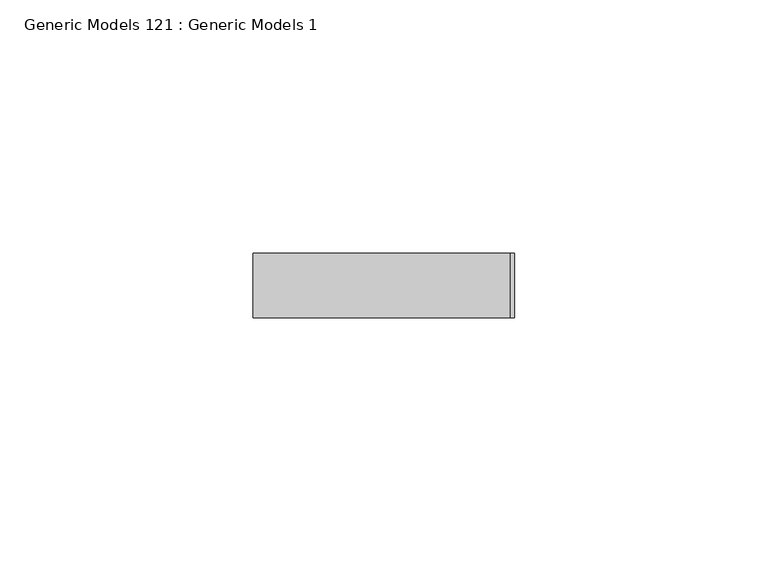
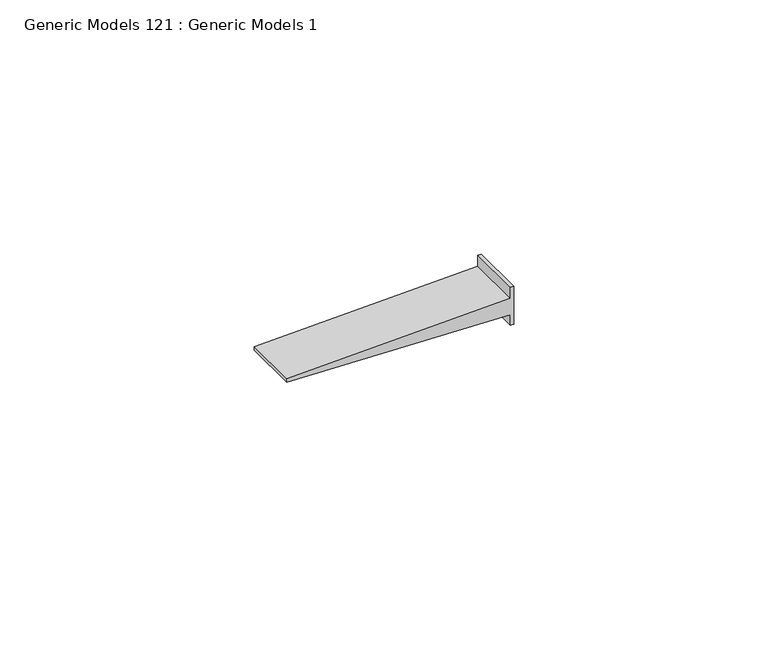
"""IFC4 building model written with IfcOpenShell, lengths in millimetres: proxy geometry, Generic Models 121 : Generic Models 1."""

import ifcopenshell
import ifcopenshell.guid

model = None  # the IFC model being written
_history = None  # IfcOwnerHistory: only IFC2X3 demands one
_inside = {}  # id of a spatial element -> (the spatial element, [elements in it])
_under = {}  # id of a project, library or spatial element -> (it, [spatial elements below it])
_declared = {}  # id of a project -> (the project, [libraries it declares])
_typed = {}  # id of a type object -> (the type object, [elements of that type])
_made_of = {}  # id of a material, layer set ... -> (it, [elements and type objects made of it])


def new_model(schema):
    """Start an empty IFC model of exactly this schema.

    Asked for "IFC4X3", IfcOpenShell would pick the latest addendum, in which some entities
    have other attributes; the version numbers below select the first issue.
    IFC2X3 requires an IfcOwnerHistory on every rooted entity: one is made here for all.
    """
    global model, _history
    if schema == "IFC4X3":
        model = ifcopenshell.file(schema_version=(4, 3, 0, 0))
    else:
        model = ifcopenshell.file(schema=schema)
    _inside.clear()
    _under.clear()
    _declared.clear()
    _typed.clear()
    _made_of.clear()
    _history = None
    if model.schema == "IFC2X3":
        org = make("IfcOrganization", Name="unknown")
        user = make(
            "IfcPersonAndOrganization",
            ThePerson=make("IfcPerson", FamilyName="unknown"),
            TheOrganization=org,
        )
        app = make(
            "IfcApplication",
            ApplicationDeveloper=org,
            Version="unknown",
            ApplicationFullName="unknown",
            ApplicationIdentifier="unknown",
        )
        _history = make(
            "IfcOwnerHistory",
            OwningUser=user,
            OwningApplication=app,
            ChangeAction="ADDED",
            CreationDate=0,
        )
    return model


def make(cls, **values):
    """One entity of the class cls with the attributes given. An attribute that is None is left unset."""
    return model.create_entity(
        cls, **{name: value for name, value in values.items() if value is not None}
    )


def rooted(cls, **values):
    """An entity with a GlobalId (a new one), such as an element, a storey or a relation."""
    return make(cls, GlobalId=ifcopenshell.guid.new(), OwnerHistory=_history, **values)


def si_unit(unit_type, name, prefix=None):
    """IfcSIUnit, for example si_unit("LENGTHUNIT", "METRE", prefix="MILLI")."""
    return make("IfcSIUnit", UnitType=unit_type, Prefix=prefix, Name=name)


def assignment(units):
    """IfcUnitAssignment: the units of a project."""
    return None if units is None else make("IfcUnitAssignment", Units=units)


def point(xyz):
    """IfcCartesianPoint."""
    return None if xyz is None else make("IfcCartesianPoint", Coordinates=xyz)


def direction(xyz):
    """IfcDirection."""
    return None if xyz is None else make("IfcDirection", DirectionRatios=xyz)


def frame(location, z_axis=None, x_axis=None):
    """IfcAxis2Placement3D, a coordinate frame: its origin and axes. An axis left out is left unset."""
    return make(
        "IfcAxis2Placement3D",
        Location=point(location),
        Axis=direction(z_axis),
        RefDirection=direction(x_axis),
    )


def origin():
    """The frame at (0, 0, 0) with its axes left unset."""
    return frame((0.0, 0.0, 0.0))


def place(relative_to, where):
    """IfcLocalPlacement: puts the frame where relative to a parent placement (None: the world)."""
    return make(
        "IfcLocalPlacement", PlacementRelTo=relative_to, RelativePlacement=where
    )


def context(
    kind, dimensions, precision=None, world=None, true_north=None, identifier=None
):
    """IfcGeometricRepresentationContext, for example the 3D "Model" context."""
    return make(
        "IfcGeometricRepresentationContext",
        ContextIdentifier=identifier,
        ContextType=kind,
        CoordinateSpaceDimension=dimensions,
        Precision=precision,
        WorldCoordinateSystem=world,
        TrueNorth=true_north,
    )


def project(units=None, contexts=None):
    """IfcProject with its units and contexts."""
    return rooted(
        "IfcProject",
        Name="project",
        RepresentationContexts=contexts,
        UnitsInContext=assignment(units),
    )


def spatial(cls, under=None, at=None, **own):
    """A site, building, storey or space (cls), placed at a placement, below another one or the project."""
    s = rooted(cls, ObjectPlacement=at, **own)
    if under is not None:
        _under.setdefault(under.id(), (under, []))[1].append(s)
    return s


def polyline(points):
    """IfcPolyline through the points."""
    return make("IfcPolyline", Points=[point(p) for p in points])


def outline(outer, holes=None, kind="AREA"):
    """IfcArbitraryClosedProfileDef: a profile drawn as a closed curve; with holes, ...WithVoids."""
    if holes is None:
        return make("IfcArbitraryClosedProfileDef", ProfileType=kind, OuterCurve=outer)
    return make(
        "IfcArbitraryProfileDefWithVoids",
        ProfileType=kind,
        OuterCurve=outer,
        InnerCurves=holes,
    )


def extrude(swept, where, along, depth):
    """IfcExtrudedAreaSolid: the profile swept, set in the frame where, extruded along a direction by depth."""
    return make(
        "IfcExtrudedAreaSolid",
        SweptArea=swept,
        Position=where,
        ExtrudedDirection=direction(along),
        Depth=depth,
    )


def shape(context_of_items, identifier, shape_type, items):
    """IfcShapeRepresentation: the items that make up one representation, for example the "Body"."""
    return make(
        "IfcShapeRepresentation",
        ContextOfItems=context_of_items,
        RepresentationIdentifier=identifier,
        RepresentationType=shape_type,
        Items=items,
    )


def source(mapping_origin, context_of_items, identifier, shape_type, items):
    """IfcRepresentationMap: a shape defined once, which mapped items show again and again."""
    return make(
        "IfcRepresentationMap",
        MappingOrigin=mapping_origin,
        MappedRepresentation=shape(context_of_items, identifier, shape_type, items),
    )


def transform(
    local_origin,
    x_axis=None,
    y_axis=None,
    z_axis=None,
    scale=None,
    scale2=None,
    scale3=None,
    uniform=True,
):
    """IfcCartesianTransformationOperator3D, or its non-uniform kind. x_axis, y_axis, z_axis: its Axis1, 2, 3."""
    if uniform:
        return make(
            "IfcCartesianTransformationOperator3D",
            Axis1=direction(x_axis),
            Axis2=direction(y_axis),
            LocalOrigin=point(local_origin),
            Scale=scale,
            Axis3=direction(z_axis),
        )
    return make(
        "IfcCartesianTransformationOperator3DnonUniform",
        Axis1=direction(x_axis),
        Axis2=direction(y_axis),
        LocalOrigin=point(local_origin),
        Scale=scale,
        Axis3=direction(z_axis),
        Scale2=scale2,
        Scale3=scale3,
    )


def mapped(mapping_source, mapping_target):
    """IfcMappedItem: shows the shape of a source again, moved by a transform."""
    return make(
        "IfcMappedItem", MappingSource=mapping_source, MappingTarget=mapping_target
    )


def made_of(thing, what):
    """Note that an element or type object is made of a material, layer set ...; save() writes the relation."""
    if what is not None:
        _made_of.setdefault(what.id(), (what, []))[1].append(thing)
    return thing


def element(
    cls,
    number,
    at=None,
    inside=None,
    cuts=None,
    type_object=None,
    material=None,
    context=None,
    identifier="Body",
    shape_type=None,
    held_by="IfcProductDefinitionShape",
    body=None,
    shapes=None,
    **own,
):
    """One element of the class cls, such as IfcWall. Its Tag is "e" and its number.

    at: its placement. inside: the storey or other place that contains it. cuts: it is an
    opening in that element (IfcRelVoidsElement). A single representation is given by context,
    identifier, shape_type and body (its items); several are given by shapes. held_by: the class
    of the entity that holds the representations. save() writes the other relations.
    """
    e = rooted(cls, Tag="e%d" % number, ObjectPlacement=at, **own)
    if body is not None:
        shapes = [shape(context, identifier, shape_type, body)]
    if shapes is not None:
        e.Representation = make(held_by, Representations=shapes)
    if inside is not None:
        _inside.setdefault(inside.id(), (inside, []))[1].append(e)
    if cuts is not None:
        rooted(
            "IfcRelVoidsElement", RelatingBuildingElement=cuts, RelatedOpeningElement=e
        )
    if type_object is not None:
        _typed.setdefault(type_object.id(), (type_object, []))[1].append(e)
    return made_of(e, material)


def aggregate(whole, parts):
    """IfcRelAggregates: a whole, such as a stair, and the parts it consists of."""
    return rooted("IfcRelAggregates", RelatingObject=whole, RelatedObjects=parts)


def save(model, path):
    """Write the relations noted so far, then the file.

    IfcRelAggregates (storeys below a building ...), IfcRelContainedInSpatialStructure (elements
    in a storey), IfcRelDefinesByType, IfcRelAssociatesMaterial and IfcRelDeclares: one each for
    every whole, place, type object, material and project.
    """
    for whole, parts in _under.values():
        aggregate(whole, parts)
    for where, things in _inside.values():
        rooted(
            "IfcRelContainedInSpatialStructure",
            RelatedElements=things,
            RelatingStructure=where,
        )
    for kind, things in _typed.values():
        rooted("IfcRelDefinesByType", RelatedObjects=things, RelatingType=kind)
    for what, things in _made_of.values():
        rooted("IfcRelAssociatesMaterial", RelatedObjects=things, RelatingMaterial=what)
    for by, libraries in _declared.values():
        rooted("IfcRelDeclares", RelatingContext=by, RelatedDefinitions=libraries)
    model.write(path)


def generic_models_121_generic_models_1_ae7d0063(model_context):
    return source(origin(), model_context, "Body", "SweptSolid", [
        extrude(outline(polyline([(2183.633033, 46952.5423031), (2183.633033, 46951.7485531), (2181.0831694, 46951.7485531), (2179.4857803, 46900.9485531), (2178.6870857, 46900.9485531), (2177.0896966, 46951.7485531), (2174.539833, 46951.7485531), (2174.539833, 46952.5423031), (2183.633033, 46952.5423031)])), frame((0.0, 565.15, 0.0), z_axis=(0.0, 1.0, 0.0), x_axis=(0.0, 0.0, 1.0)), (0.0, 0.0, 1.0), 12.7),
    ])


if __name__ == "__main__":
    model = new_model("IFC4")
    model_context = context("Model", 3, world=origin())
    ifc_project = project(units=[si_unit("LENGTHUNIT", "METRE", prefix="MILLI")], contexts=[model_context])
    site = spatial("IfcSite", under=ifc_project)
    building = spatial("IfcBuilding", under=site)
    placement = place(None, origin())
    generic_models_121_generic_models_1_shape = generic_models_121_generic_models_1_ae7d0063(model_context)
    element("IfcBuildingElementProxy", 1, Name="Generic Models 121 : Generic Models 1", ObjectType="Generic Models 121 : Generic Models 1", at=placement, inside=building, context=model_context, shape_type="MappedRepresentation", body=[
        mapped(generic_models_121_generic_models_1_shape, transform((0.0, 0.0, 0.0), x_axis=(1.0, 0.0, 0.0), y_axis=(0.0, 1.0, 0.0), z_axis=(0.0, 0.0, 1.0))),
    ])
    save(model, "model.ifc")

# Revit data of these elements
# Element 1 (IfcBuildingElementProxy, "Generic Models 121 : Generic Models 1")
#   Materials on its faces: "ATTACH GYPSUM BOARD TO STUDS AND NOT TO TOP TRACK"
# Materials
#   "ATTACH GYPSUM BOARD TO STUDS AND NOT TO TOP TRACK": class "Generic", colour RGB 48 48 48, transparency 0, Cost = 0
